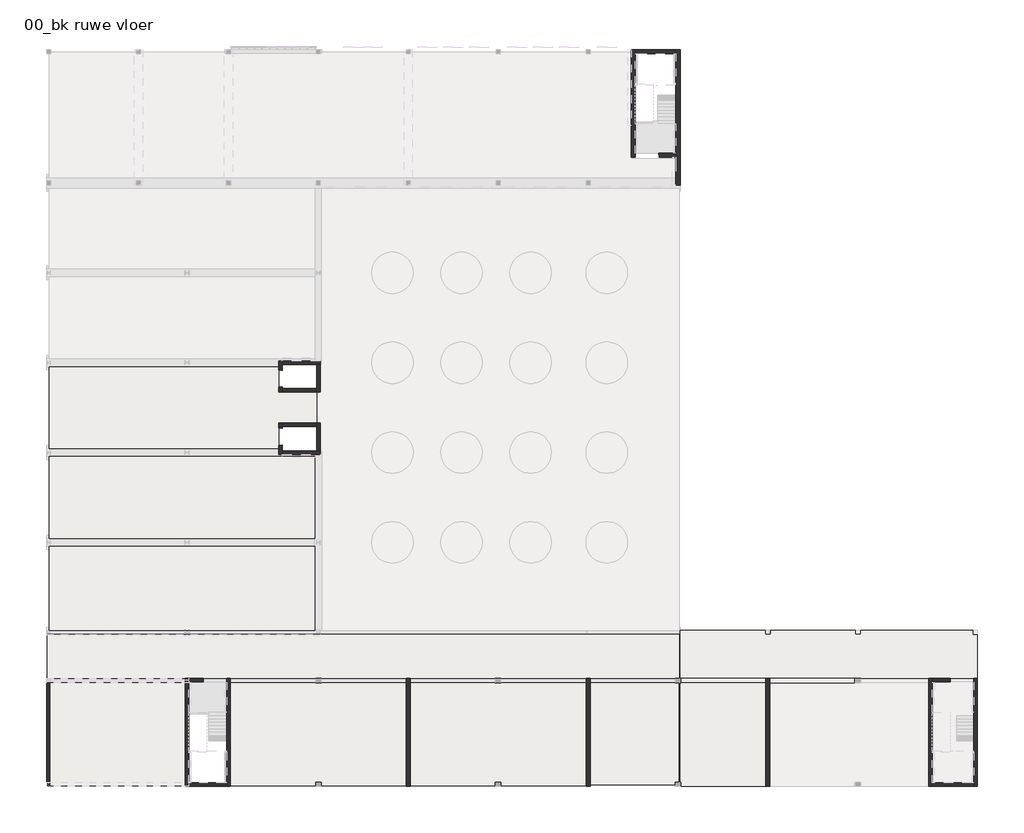
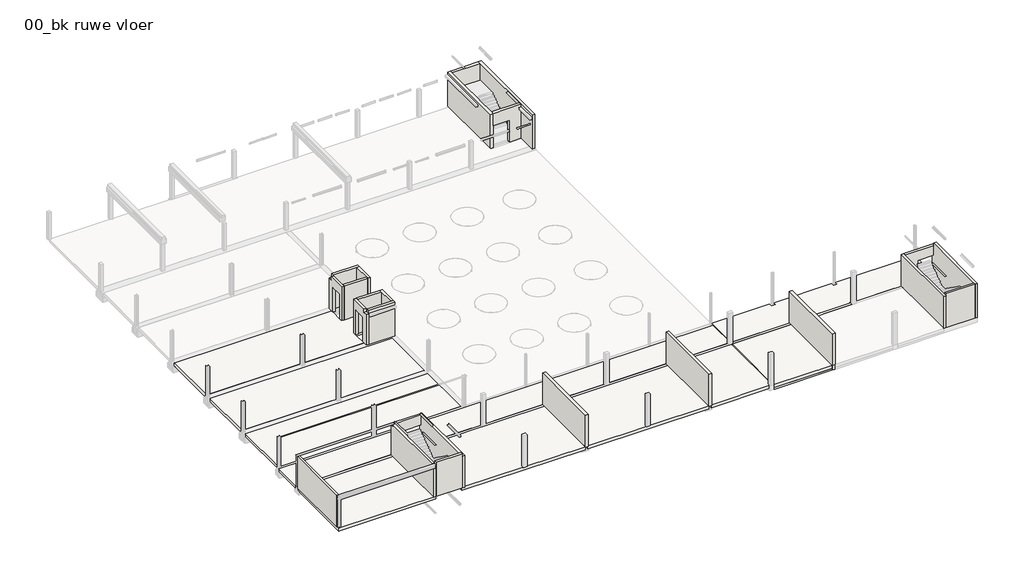
# One storey, part 1 of 6: 24 walls, 18 slabs.
"""IFC4 building model written with IfcOpenShell, lengths in millimetres."""

import ifcopenshell
import ifcopenshell.guid

model = None  # the IFC model being written
_history = None  # IfcOwnerHistory: only IFC2X3 demands one
_inside = {}  # id of a spatial element -> (the spatial element, [elements in it])
_under = {}  # id of a project, library or spatial element -> (it, [spatial elements below it])
_declared = {}  # id of a project -> (the project, [libraries it declares])
_typed = {}  # id of a type object -> (the type object, [elements of that type])
_made_of = {}  # id of a material, layer set ... -> (it, [elements and type objects made of it])


def new_model(schema):
    """Start an empty IFC model of exactly this schema.

    Asked for "IFC4X3", IfcOpenShell would pick the latest addendum, in which some entities
    have other attributes; the version numbers below select the first issue.
    IFC2X3 requires an IfcOwnerHistory on every rooted entity: one is made here for all.
    """
    global model, _history
    if schema == "IFC4X3":
        model = ifcopenshell.file(schema_version=(4, 3, 0, 0))
    else:
        model = ifcopenshell.file(schema=schema)
    _inside.clear()
    _under.clear()
    _declared.clear()
    _typed.clear()
    _made_of.clear()
    _history = None
    if model.schema == "IFC2X3":
        org = make("IfcOrganization", Name="unknown")
        user = make(
            "IfcPersonAndOrganization",
            ThePerson=make("IfcPerson", FamilyName="unknown"),
            TheOrganization=org,
        )
        app = make(
            "IfcApplication",
            ApplicationDeveloper=org,
            Version="unknown",
            ApplicationFullName="unknown",
            ApplicationIdentifier="unknown",
        )
        _history = make(
            "IfcOwnerHistory",
            OwningUser=user,
            OwningApplication=app,
            ChangeAction="ADDED",
            CreationDate=0,
        )
    return model


def make(cls, **values):
    """One entity of the class cls with the attributes given. An attribute that is None is left unset."""
    return model.create_entity(
        cls, **{name: value for name, value in values.items() if value is not None}
    )


def rooted(cls, **values):
    """An entity with a GlobalId (a new one), such as an element, a storey or a relation."""
    return make(cls, GlobalId=ifcopenshell.guid.new(), OwnerHistory=_history, **values)


def si_unit(unit_type, name, prefix=None):
    """IfcSIUnit, for example si_unit("LENGTHUNIT", "METRE", prefix="MILLI")."""
    return make("IfcSIUnit", UnitType=unit_type, Prefix=prefix, Name=name)


def assignment(units):
    """IfcUnitAssignment: the units of a project."""
    return None if units is None else make("IfcUnitAssignment", Units=units)


def point(xyz):
    """IfcCartesianPoint."""
    return None if xyz is None else make("IfcCartesianPoint", Coordinates=xyz)


def direction(xyz):
    """IfcDirection."""
    return None if xyz is None else make("IfcDirection", DirectionRatios=xyz)


def frame(location, z_axis=None, x_axis=None):
    """IfcAxis2Placement3D, a coordinate frame: its origin and axes. An axis left out is left unset."""
    return make(
        "IfcAxis2Placement3D",
        Location=point(location),
        Axis=direction(z_axis),
        RefDirection=direction(x_axis),
    )


def origin():
    """The frame at (0, 0, 0) with its axes left unset."""
    return frame((0.0, 0.0, 0.0))


def place(relative_to, where):
    """IfcLocalPlacement: puts the frame where relative to a parent placement (None: the world)."""
    return make(
        "IfcLocalPlacement", PlacementRelTo=relative_to, RelativePlacement=where
    )


def context(
    kind, dimensions, precision=None, world=None, true_north=None, identifier=None
):
    """IfcGeometricRepresentationContext, for example the 3D "Model" context."""
    return make(
        "IfcGeometricRepresentationContext",
        ContextIdentifier=identifier,
        ContextType=kind,
        CoordinateSpaceDimension=dimensions,
        Precision=precision,
        WorldCoordinateSystem=world,
        TrueNorth=true_north,
    )


def project(units=None, contexts=None):
    """IfcProject with its units and contexts."""
    return rooted(
        "IfcProject",
        Name="project",
        RepresentationContexts=contexts,
        UnitsInContext=assignment(units),
    )


def spatial(cls, under=None, at=None, **own):
    """A site, building, storey or space (cls), placed at a placement, below another one or the project."""
    s = rooted(cls, ObjectPlacement=at, **own)
    if under is not None:
        _under.setdefault(under.id(), (under, []))[1].append(s)
    return s


def polyline(points):
    """IfcPolyline through the points."""
    return make("IfcPolyline", Points=[point(p) for p in points])


def outline(outer, holes=None, kind="AREA"):
    """IfcArbitraryClosedProfileDef: a profile drawn as a closed curve; with holes, ...WithVoids."""
    if holes is None:
        return make("IfcArbitraryClosedProfileDef", ProfileType=kind, OuterCurve=outer)
    return make(
        "IfcArbitraryProfileDefWithVoids",
        ProfileType=kind,
        OuterCurve=outer,
        InnerCurves=holes,
    )


def extrude(swept, where, along, depth):
    """IfcExtrudedAreaSolid: the profile swept, set in the frame where, extruded along a direction by depth."""
    return make(
        "IfcExtrudedAreaSolid",
        SweptArea=swept,
        Position=where,
        ExtrudedDirection=direction(along),
        Depth=depth,
    )


def faces_of(points, faces, orient=None, outer=None):
    """IfcFace entities. A face is a list of loops; a loop is a list of indices into points, from 0.

    orient and outer hold one flag for each loop. By default every Orientation is true, the
    first loop of a face is its IfcFaceOuterBound and the others are IfcFaceBound.
    """
    made = []
    for i, loops in enumerate(faces):
        bounds = []
        for j, loop in enumerate(loops):
            is_outer = j == 0 if outer is None else outer[i][j]
            bounds.append(
                make(
                    "IfcFaceOuterBound" if is_outer else "IfcFaceBound",
                    Bound=make("IfcPolyLoop", Polygon=[points[k] for k in loop]),
                    Orientation=True if orient is None else orient[i][j],
                )
            )
        made.append(make("IfcFace", Bounds=bounds))
    return made


def faceted_brep(points, faces, orient=None, outer=None, voids=None):
    """IfcFacetedBrep: a solid bounded by flat faces; with voids (closed shells), ...WithVoids."""
    shared = [point(p) for p in points]
    hull = make("IfcClosedShell", CfsFaces=faces_of(shared, faces, orient, outer))
    if voids is None:
        return make("IfcFacetedBrep", Outer=hull)
    return make(
        "IfcFacetedBrepWithVoids",
        Outer=hull,
        Voids=[
            make(cls, CfsFaces=faces_of(shared, fs, o, b)) for cls, fs, o, b in voids
        ],
    )


def shape(context_of_items, identifier, shape_type, items):
    """IfcShapeRepresentation: the items that make up one representation, for example the "Body"."""
    return make(
        "IfcShapeRepresentation",
        ContextOfItems=context_of_items,
        RepresentationIdentifier=identifier,
        RepresentationType=shape_type,
        Items=items,
    )


def made_of(thing, what):
    """Note that an element or type object is made of a material, layer set ...; save() writes the relation."""
    if what is not None:
        _made_of.setdefault(what.id(), (what, []))[1].append(thing)
    return thing


def element(
    cls,
    number,
    at=None,
    inside=None,
    cuts=None,
    type_object=None,
    material=None,
    context=None,
    identifier="Body",
    shape_type=None,
    held_by="IfcProductDefinitionShape",
    body=None,
    shapes=None,
    **own,
):
    """One element of the class cls, such as IfcWall. Its Tag is "e" and its number.

    at: its placement. inside: the storey or other place that contains it. cuts: it is an
    opening in that element (IfcRelVoidsElement). A single representation is given by context,
    identifier, shape_type and body (its items); several are given by shapes. held_by: the class
    of the entity that holds the representations. save() writes the other relations.
    """
    e = rooted(cls, Tag="e%d" % number, ObjectPlacement=at, **own)
    if body is not None:
        shapes = [shape(context, identifier, shape_type, body)]
    if shapes is not None:
        e.Representation = make(held_by, Representations=shapes)
    if inside is not None:
        _inside.setdefault(inside.id(), (inside, []))[1].append(e)
    if cuts is not None:
        rooted(
            "IfcRelVoidsElement", RelatingBuildingElement=cuts, RelatedOpeningElement=e
        )
    if type_object is not None:
        _typed.setdefault(type_object.id(), (type_object, []))[1].append(e)
    return made_of(e, material)


def aggregate(whole, parts):
    """IfcRelAggregates: a whole, such as a stair, and the parts it consists of."""
    return rooted("IfcRelAggregates", RelatingObject=whole, RelatedObjects=parts)


def save(model, path):
    """Write the relations noted so far, then the file.

    IfcRelAggregates (storeys below a building ...), IfcRelContainedInSpatialStructure (elements
    in a storey), IfcRelDefinesByType, IfcRelAssociatesMaterial and IfcRelDeclares: one each for
    every whole, place, type object, material and project.
    """
    for whole, parts in _under.values():
        aggregate(whole, parts)
    for where, things in _inside.values():
        rooted(
            "IfcRelContainedInSpatialStructure",
            RelatedElements=things,
            RelatingStructure=where,
        )
    for kind, things in _typed.values():
        rooted("IfcRelDefinesByType", RelatedObjects=things, RelatingType=kind)
    for what, things in _made_of.values():
        rooted("IfcRelAssociatesMaterial", RelatedObjects=things, RelatingMaterial=what)
    for by, libraries in _declared.values():
        rooted("IfcRelDeclares", RelatingContext=by, RelatedDefinitions=libraries)
    model.write(path)


model = new_model("IFC4")

# Units and contexts
model_context = context("Model", 3, world=origin())
ifc_project = project(units=[si_unit("LENGTHUNIT", "METRE", prefix="MILLI")], contexts=[model_context])

# Site, building, storey
site = spatial("IfcSite", under=ifc_project)
building = spatial("IfcBuilding", under=site)
storey = spatial("IfcBuildingStorey", under=building, Name="00_bk ruwe vloer", Elevation=-70.0)

# Slabs
placement = place(None, origin())
element("IfcSlab", 1, ObjectType="NLRS_23_FL_isolatieplaatvloer 320_gen_rsf", at=placement, inside=storey, context=model_context, shape_type="Brep", body=[
    faceted_brep([(52150.0, 7650.0, -390.0), (52150.0, 11150.0, -390.0), (58300.0, 11150.0, -390.0), (58300.0, 10850.0, -390.0), (58700.0, 10850.0, -390.0), (58700.0, 11150.0, -390.0), (64800.0, 11150.0, -390.0), (64800.0, 10850.0, -390.0), (65200.0, 10850.0, -390.0), (65200.0, 11150.0, -390.0), (73300.0, 11150.0, -390.0), (73300.0, 10800.0, -390.0), (73650.0, 10800.0, -390.0), (73650.0, 7650.0, -390.0), (65250.0, 7650.0, -390.0), (65250.0, 7700.0, -390.0), (64750.0, 7700.0, -390.0), (64750.0, 7650.0, -390.0), (52150.0, 7650.0, -70.0), (64750.0, 7650.0, -70.0), (64750.0, 7700.0, -70.0), (65250.0, 7700.0, -70.0), (65250.0, 7650.0, -70.0), (73650.0, 7650.0, -70.0), (73650.0, 10800.0, -70.0), (73300.0, 10800.0, -70.0), (73300.0, 11150.0, -70.0), (65200.0, 11150.0, -70.0), (65200.0, 10850.0, -70.0), (64800.0, 10850.0, -70.0), (64800.0, 11150.0, -70.0), (58700.0, 11150.0, -70.0), (58700.0, 10850.0, -70.0), (58300.0, 10850.0, -70.0), (58300.0, 11150.0, -70.0), (52150.0, 11150.0, -70.0), (52150.0, 10850.0, -70.0)], [[[0, 1, 2, 3, 4, 5, 6, 7, 8, 9, 10, 11, 12, 13, 14, 15, 16, 17]], [[18, 19, 20, 21, 22, 23, 24, 25, 26, 27, 28, 29, 30, 31, 32, 33, 34, 35, 36]], [[1, 0, 18, 36, 35]], [[10, 9, 27, 26]], [[13, 12, 24, 23]], [[0, 17, 19, 18]], [[14, 13, 23, 22]], [[15, 14, 22, 21]], [[16, 15, 21, 20]], [[17, 16, 20, 19]], [[2, 1, 35, 34]], [[3, 2, 34, 33]], [[4, 3, 33, 32]], [[5, 4, 32, 31]], [[6, 5, 31, 30]], [[7, 6, 30, 29]], [[8, 7, 29, 28]], [[9, 8, 28, 27]], [[11, 10, 26, 25]], [[12, 11, 25, 24]]]),
])
element("IfcSlab", 2, ObjectType="NLRS_23_FL_breedplaat 320_gen_rsf", at=placement, inside=storey, context=model_context, shape_type="Brep", body=[
    faceted_brep([(6410.0, 7350.0, -390.0), (16375.0, 7350.0, -390.0), (16625.0, 7350.0, -390.0), (16625.0, 150.0, -390.0), (16625.0, -90.0, -390.0), (6650.0, -90.0, -390.0), (6410.0, -90.0, -390.0), (6410.0, 7150.0, -390.0), (16400.0, 125.0, -390.0), (16400.0, 7175.0, -390.0), (6625.0, 7175.0, -390.0), (6625.0, 125.0, -390.0), (16625.0, 7350.0, -70.0), (6410.0, 7350.0, -70.0), (6410.0, -90.0, -70.0), (6650.0, -90.0, -70.0), (16625.0, -90.0, -70.0), (16625.0, 150.0, -70.0), (6625.0, 7175.0, -330.0), (16400.0, 7175.0, -330.0), (16400.0, 125.0, -330.0), (6625.0, 125.0, -330.0)], [[[0, 1, 2, 3, 4, 5, 6, 7], [8, 9, 10, 11]], [[12, 13, 14, 15, 16, 17]], [[2, 1, 0, 13, 12]], [[4, 3, 2, 12, 17, 16]], [[6, 5, 4, 16, 15, 14]], [[0, 7, 6, 14, 13]], [[18, 19, 20, 21]], [[20, 19, 9, 8]], [[21, 20, 8, 11]], [[18, 21, 11, 10]], [[19, 18, 10, 9]]]),
])
element("IfcSlab", 3, ObjectType="NLRS_23_FL_breedplaat 320_gen_rsf", at=placement, inside=storey, context=model_context, shape_type="Brep", body=[
    faceted_brep([(52090.0, 10850.0, -390.0), (52090.0, 10650.0, -390.0), (52090.0, 7850.0, -390.0), (52090.0, 7650.0, -390.0), (19375.0, 7650.0, -390.0), (16625.0, 7650.0, -390.0), (16375.0, 7650.0, -390.0), (6410.0, 7650.0, -390.0), (6410.0, 7850.0, -390.0), (6410.0, 10650.0, -390.0), (6410.0, 10850.0, -390.0), (51875.0, 7825.0, -390.0), (51875.0, 10675.0, -390.0), (6625.0, 10675.0, -390.0), (6625.0, 7825.0, -390.0), (52090.0, 7650.0, -70.0), (52090.0, 10850.0, -70.0), (6410.0, 10850.0, -70.0), (6410.0, 7650.0, -70.0), (16625.0, 7650.0, -70.0), (19375.0, 7650.0, -70.0), (6625.0, 10675.0, -330.0), (51875.0, 10675.0, -330.0), (51875.0, 7825.0, -330.0), (6625.0, 7825.0, -330.0)], [[[0, 1, 2, 3, 4, 5, 6, 7, 8, 9, 10], [11, 12, 13, 14]], [[15, 16, 17, 18, 19, 20]], [[3, 2, 1, 0, 16, 15]], [[7, 6, 5, 4, 3, 15, 20, 19, 18]], [[10, 9, 8, 7, 18, 17]], [[0, 10, 17, 16]], [[21, 22, 23, 24]], [[23, 22, 12, 11]], [[24, 23, 11, 14]], [[21, 24, 14, 13]], [[22, 21, 13, 12]]]),
])
element("IfcSlab", 4, ObjectType="NLRS_23_FL_isolatieplaatvloer 320_gen_rsf", at=placement, inside=storey, context=model_context, shape_type="Brep", body=[
    faceted_brep([(25750.0, 17200.0, -390.0), (25750.0, 11350.0, -390.0), (25750.0, 11150.0, -390.0), (6550.0, 11150.0, -390.0), (6550.0, 11350.0, -390.0), (6550.0, 17000.0, -390.0), (6550.0, 17200.0, -390.0), (25500.0, 17200.0, -390.0), (25550.0, 17200.0, -390.0), (25700.0, 17200.0, -390.0), (25750.0, 17200.0, -70.0), (25700.0, 17200.0, -70.0), (6550.0, 17200.0, -70.0), (6550.0, 11150.0, -70.0), (25750.0, 11150.0, -70.0)], [[[0, 1, 2, 3, 4, 5, 6, 7, 8, 9]], [[10, 11, 12, 13, 14]], [[2, 1, 0, 10, 14]], [[3, 2, 14, 13]], [[6, 5, 4, 3, 13, 12]], [[0, 9, 8, 7, 6, 12, 11, 10]]]),
])
element("IfcSlab", 5, ObjectType="NLRS_23_FL_isolatieplaatvloer 320_gen_rsf", at=placement, inside=storey, context=model_context, shape_type="Brep", body=[
    faceted_brep([(25750.0, 23700.0, -390.0), (25750.0, 17800.0, -390.0), (25700.0, 17800.0, -390.0), (25550.0, 17800.0, -390.0), (25500.0, 17800.0, -390.0), (6550.0, 17800.0, -390.0), (6550.0, 18000.0, -390.0), (6550.0, 23500.0, -390.0), (6550.0, 23700.0, -390.0), (25500.0, 23700.0, -390.0), (25550.0, 23700.0, -390.0), (25700.0, 23700.0, -390.0), (25750.0, 23700.0, -70.0), (25700.0, 23700.0, -70.0), (6550.0, 23700.0, -70.0), (6550.0, 17800.0, -70.0), (25700.0, 17800.0, -70.0), (25750.0, 17800.0, -70.0)], [[[0, 1, 2, 3, 4, 5, 6, 7, 8, 9, 10, 11]], [[12, 13, 14, 15, 16, 17]], [[1, 0, 12, 17]], [[5, 4, 3, 2, 1, 17, 16, 15]], [[8, 7, 6, 5, 15, 14]], [[0, 11, 10, 9, 8, 14, 13, 12]]]),
])
element("IfcSlab", 6, ObjectType="NLRS_23_FL_isolatieplaatvloer 320_gen_rsf", at=placement, inside=storey, context=model_context, shape_type="Brep", body=[
    faceted_brep([(23125.0, 30200.0, -390.0), (23125.0, 30000.0, -390.0), (23125.0, 28475.0, -390.0), (23375.0, 28475.0, -390.0), (25875.0, 28475.0, -390.0), (25875.0, 28375.0, -390.0), (25875.0, 26125.0, -390.0), (25875.0, 26025.0, -390.0), (23375.0, 26025.0, -390.0), (23125.0, 26025.0, -390.0), (23125.0, 24500.0, -390.0), (23125.0, 24300.0, -390.0), (6550.0, 24300.0, -390.0), (6550.0, 24500.0, -390.0), (6550.0, 30000.0, -390.0), (6550.0, 30200.0, -390.0), (23125.0, 30200.0, -70.0), (6550.0, 30200.0, -70.0), (6550.0, 24300.0, -70.0), (23125.0, 24300.0, -70.0), (23125.0, 26025.0, -70.0), (23375.0, 26025.0, -70.0), (25875.0, 26025.0, -70.0), (25875.0, 28475.0, -70.0), (23375.0, 28475.0, -70.0), (23125.0, 28475.0, -70.0)], [[[0, 1, 2, 3, 4, 5, 6, 7, 8, 9, 10, 11, 12, 13, 14, 15]], [[16, 17, 18, 19, 20, 21, 22, 23, 24, 25]], [[2, 1, 0, 16, 25]], [[12, 11, 19, 18]], [[15, 14, 13, 12, 18, 17]], [[0, 15, 17, 16]], [[4, 3, 2, 25, 24, 23]], [[7, 6, 5, 4, 23, 22]], [[9, 8, 7, 22, 21, 20]], [[11, 10, 9, 20, 19]]]),
])
element("IfcSlab", 7, ObjectType="NLRS_23_FL_breedplaat 320_gen_rsf", at=placement, inside=storey, context=model_context, shape_type="Brep", body=[
    faceted_brep([(32350.0, 7350.0, -390.0), (32350.0, 150.0, -390.0), (32350.0, -90.0, -390.0), (19375.0, -90.0, -390.0), (19375.0, 150.0, -390.0), (19375.0, 7350.0, -390.0), (32175.0, 125.0, -390.0), (32175.0, 7175.0, -390.0), (19600.0, 7175.0, -390.0), (19600.0, 125.0, -390.0), (32350.0, -90.0, -70.0), (32350.0, 150.0, -70.0), (32350.0, 7350.0, -70.0), (19375.0, 7350.0, -70.0), (19375.0, 150.0, -70.0), (19375.0, -90.0, -70.0), (19600.0, 7175.0, -330.0), (32175.0, 7175.0, -330.0), (32175.0, 125.0, -330.0), (19600.0, 125.0, -330.0)], [[[0, 1, 2, 3, 4, 5], [6, 7, 8, 9]], [[10, 11, 12, 13, 14, 15]], [[2, 1, 0, 12, 11, 10]], [[3, 2, 10, 15]], [[5, 4, 3, 15, 14, 13]], [[0, 5, 13, 12]], [[16, 17, 18, 19]], [[18, 17, 7, 6]], [[19, 18, 6, 9]], [[16, 19, 9, 8]], [[17, 16, 8, 7]]]),
])
element("IfcSlab", 8, ObjectType="NLRS_23_FL_breedplaat 320_gen_rsf", at=placement, inside=storey, context=model_context, shape_type="Brep", body=[
    faceted_brep([(45350.0, 7350.0, -390.0), (45350.0, 7150.0, -390.0), (45350.0, 150.0, -390.0), (45350.0, -90.0, -390.0), (32650.0, -90.0, -390.0), (32650.0, 150.0, -390.0), (32650.0, 7150.0, -390.0), (32650.0, 7350.0, -390.0), (45175.0, 125.0, -390.0), (45175.0, 7175.0, -390.0), (32825.0, 7175.0, -390.0), (32825.0, 125.0, -390.0), (45350.0, -90.0, -70.0), (45350.0, 150.0, -70.0), (45350.0, 7350.0, -70.0), (32650.0, 7350.0, -70.0), (32650.0, 150.0, -70.0), (32650.0, -90.0, -70.0), (32825.0, 7175.0, -330.0), (45175.0, 7175.0, -330.0), (45175.0, 125.0, -330.0), (32825.0, 125.0, -330.0)], [[[0, 1, 2, 3, 4, 5, 6, 7], [8, 9, 10, 11]], [[12, 13, 14, 15, 16, 17]], [[3, 2, 1, 0, 14, 13, 12]], [[4, 3, 12, 17]], [[7, 6, 5, 4, 17, 16, 15]], [[0, 7, 15, 14]], [[18, 19, 20, 21]], [[20, 19, 9, 8]], [[21, 20, 8, 11]], [[18, 21, 11, 10]], [[19, 18, 10, 9]]]),
])
element("IfcSlab", 9, ObjectType="NLRS_23_FL_breedplaat 320_gen_rsf", at=placement, inside=storey, context=model_context, shape_type="Brep", body=[
    faceted_brep([(52050.0, 7350.0, -390.0), (52050.0, 7150.0, -390.0), (52050.0, 150.0, -390.0), (52050.0, -50.0, -390.0), (51750.0, -50.0, -390.0), (45650.0, -50.0, -390.0), (45650.0, 150.0, -390.0), (45650.0, 7150.0, -390.0), (45650.0, 7350.0, -390.0), (51875.0, 125.0, -390.0), (51875.0, 7175.0, -390.0), (45825.0, 7175.0, -390.0), (45825.0, 125.0, -390.0), (52050.0, -50.0, -70.0), (52050.0, 150.0, -70.0), (52050.0, 7350.0, -70.0), (45650.0, 7350.0, -70.0), (45650.0, 150.0, -70.0), (45650.0, -50.0, -70.0), (51750.0, -50.0, -70.0), (45825.0, 7175.0, -330.0), (51875.0, 7175.0, -330.0), (51875.0, 125.0, -330.0), (45825.0, 125.0, -330.0)], [[[0, 1, 2, 3, 4, 5, 6, 7, 8], [9, 10, 11, 12]], [[13, 14, 15, 16, 17, 18, 19]], [[3, 2, 1, 0, 15, 14, 13]], [[5, 4, 3, 13, 19, 18]], [[8, 7, 6, 5, 18, 17, 16]], [[0, 8, 16, 15]], [[20, 21, 22, 23]], [[22, 21, 10, 9]], [[23, 22, 9, 12]], [[20, 23, 12, 11]], [[21, 20, 11, 10]]]),
])
element("IfcSlab", 10, ObjectType="NLRS_23_FL_isolatieplaatvloer 320_gen_rsf", at=placement, inside=storey, context=model_context, shape_type="SweptSolid", body=[
    extrude(outline(polyline([(58350.0, 7350.0), (58350.0, -150.0), (52250.0, -150.0), (52250.0, 150.0), (52150.0, 150.0), (52150.0, 7350.0), (58350.0, 7350.0)])), frame((0.0, 0.0, -390.0), z_axis=(0.0, 0.0, 1.0), x_axis=(1.0, 0.0, 0.0)), (0.0, 0.0, 1.0), 320.0),
])
element("IfcSlab", 11, ObjectType="NLRS_23_FL_beton ihwg vloeraanstort 520_gen_rsf", at=placement, inside=storey, context=model_context, shape_type="Brep", body=[
    faceted_brep([(64750.0, 7650.0, -590.0), (64750.0, 7350.0, -590.0), (58650.0, 7350.0, -590.0), (58650.0, -150.0, -590.0), (58350.0, -150.0, -590.0), (58350.0, 7350.0, -590.0), (52150.0, 7350.0, -590.0), (52150.0, 7650.0, -590.0), (64750.0, 7650.0, -70.0), (52200.0, 7650.0, -70.0), (52150.0, 7650.0, -70.0), (52150.0, 7350.0, -70.0), (52200.0, 7350.0, -70.0), (58350.0, 7350.0, -70.0), (58350.0, -150.0, -70.0), (58650.0, -150.0, -70.0), (58650.0, 7350.0, -70.0), (64750.0, 7350.0, -70.0), (52150.0, 7350.0, -390.0), (52150.0, 7650.0, -390.0)], [[[0, 1, 2, 3, 4, 5, 6, 7]], [[8, 9, 10, 11, 12, 13, 14, 15, 16, 17]], [[1, 0, 8, 17]], [[2, 1, 17, 16]], [[3, 2, 16, 15]], [[4, 3, 15, 14]], [[5, 4, 14, 13]], [[6, 5, 13, 12, 11, 18]], [[7, 6, 18, 11, 10, 19]], [[0, 7, 19, 10, 9, 8]]]),
])
element("IfcSlab", 12, ObjectType="NLRS_23_FL_isolatie isolatieplaatvloer 200_gen_rsf", at=placement, inside=storey, context=model_context, shape_type="Brep", body=[
    faceted_brep([(52150.0, 7650.0, -590.0), (52150.0, 7800.0, -590.0), (52150.0, 10750.0, -590.0), (52150.0, 11150.0, -590.0), (58300.0, 11150.0, -590.0), (58300.0, 10850.0, -590.0), (58700.0, 10850.0, -590.0), (58700.0, 11150.0, -590.0), (64800.0, 11150.0, -590.0), (64800.0, 10850.0, -590.0), (65200.0, 10850.0, -590.0), (65200.0, 11150.0, -590.0), (73300.0, 11150.0, -590.0), (73300.0, 10800.0, -590.0), (73650.0, 10800.0, -590.0), (73650.0, 7650.0, -590.0), (65250.0, 7650.0, -590.0), (65250.0, 7700.0, -590.0), (64750.0, 7700.0, -590.0), (64750.0, 7650.0, -590.0), (52150.0, 7650.0, -390.0), (64750.0, 7650.0, -390.0), (64750.0, 7700.0, -390.0), (65250.0, 7700.0, -390.0), (65250.0, 7650.0, -390.0), (73650.0, 7650.0, -390.0), (73650.0, 10800.0, -390.0), (73300.0, 10800.0, -390.0), (73300.0, 11150.0, -390.0), (65200.0, 11150.0, -390.0), (65200.0, 10850.0, -390.0), (64800.0, 10850.0, -390.0), (64800.0, 11150.0, -390.0), (58700.0, 11150.0, -390.0), (58700.0, 10850.0, -390.0), (58300.0, 10850.0, -390.0), (58300.0, 11150.0, -390.0), (52150.0, 11150.0, -390.0), (52150.0, 10850.0, -390.0), (52150.0, 10650.0, -390.0), (52150.0, 7850.0, -390.0)], [[[0, 1, 2, 3, 4, 5, 6, 7, 8, 9, 10, 11, 12, 13, 14, 15, 16, 17, 18, 19]], [[20, 21, 22, 23, 24, 25, 26, 27, 28, 29, 30, 31, 32, 33, 34, 35, 36, 37, 38, 39, 40]], [[3, 2, 1, 0, 20, 40, 39, 38, 37]], [[12, 11, 29, 28]], [[15, 14, 26, 25]], [[0, 19, 21, 20]], [[16, 15, 25, 24]], [[17, 16, 24, 23]], [[18, 17, 23, 22]], [[19, 18, 22, 21]], [[4, 3, 37, 36]], [[5, 4, 36, 35]], [[6, 5, 35, 34]], [[7, 6, 34, 33]], [[8, 7, 33, 32]], [[9, 8, 32, 31]], [[10, 9, 31, 30]], [[11, 10, 30, 29]], [[13, 12, 28, 27]], [[14, 13, 27, 26]]]),
])
element("IfcSlab", 13, ObjectType="NLRS_23_FL_isolatie isolatieplaatvloer 200_gen_rsf", at=placement, inside=storey, context=model_context, shape_type="Brep", body=[
    faceted_brep([(58350.0, 7350.0, -590.0), (58350.0, -150.0, -590.0), (52250.0, -150.0, -590.0), (52250.0, 150.0, -590.0), (52150.0, 150.0, -590.0), (52150.0, 250.0, -590.0), (52150.0, 7200.0, -590.0), (52150.0, 7350.0, -590.0), (58350.0, 7350.0, -390.0), (52150.0, 7350.0, -390.0), (52150.0, 7150.0, -390.0), (52150.0, 150.0, -390.0), (52250.0, 150.0, -390.0), (52250.0, -150.0, -390.0), (58350.0, -150.0, -390.0)], [[[0, 1, 2, 3, 4, 5, 6, 7]], [[8, 9, 10, 11, 12, 13, 14]], [[1, 0, 8, 14]], [[2, 1, 14, 13]], [[7, 6, 5, 4, 11, 10, 9]], [[0, 7, 9, 8]], [[3, 2, 13, 12]], [[4, 3, 12, 11]]]),
])
element("IfcSlab", 14, ObjectType="NLRS_23_FL_breedplaat schil 60_gen_rsf", at=placement, inside=storey, context=model_context, shape_type="SweptSolid", body=[
    extrude(outline(polyline([(16400.0, 7175.0), (16400.0, 125.0), (6625.0, 125.0), (6625.0, 7175.0), (16400.0, 7175.0)])), frame((0.0, 0.0, -390.0), z_axis=(0.0, 0.0, 1.0), x_axis=(1.0, 0.0, 0.0)), (0.0, 0.0, 1.0), 60.0),
])
element("IfcSlab", 15, ObjectType="NLRS_23_FL_breedplaat schil 60_gen_rsf", at=placement, inside=storey, context=model_context, shape_type="SweptSolid", body=[
    extrude(outline(polyline([(32175.0, 7175.0), (32175.0, 125.0), (19600.0, 125.0), (19600.0, 7175.0), (32175.0, 7175.0)])), frame((0.0, 0.0, -390.0), z_axis=(0.0, 0.0, 1.0), x_axis=(1.0, 0.0, 0.0)), (0.0, 0.0, 1.0), 60.0),
])
element("IfcSlab", 16, ObjectType="NLRS_23_FL_breedplaat schil 60_gen_rsf", at=placement, inside=storey, context=model_context, shape_type="SweptSolid", body=[
    extrude(outline(polyline([(45175.0, 7175.0), (45175.0, 125.0), (32825.0, 125.0), (32825.0, 7175.0), (45175.0, 7175.0)])), frame((0.0, 0.0, -390.0), z_axis=(0.0, 0.0, 1.0), x_axis=(1.0, 0.0, 0.0)), (0.0, 0.0, 1.0), 60.0),
])
element("IfcSlab", 17, ObjectType="NLRS_23_FL_breedplaat schil 60_gen_rsf", at=placement, inside=storey, context=model_context, shape_type="SweptSolid", body=[
    extrude(outline(polyline([(51875.0, 7175.0), (51875.0, 125.0), (45825.0, 125.0), (45825.0, 7175.0), (51875.0, 7175.0)])), frame((0.0, 0.0, -390.0), z_axis=(0.0, 0.0, 1.0), x_axis=(1.0, 0.0, 0.0)), (0.0, 0.0, 1.0), 60.0),
])
element("IfcSlab", 18, ObjectType="NLRS_23_FL_breedplaat schil 60_gen_rsf", at=placement, inside=storey, context=model_context, shape_type="SweptSolid", body=[
    extrude(outline(polyline([(51875.0, 10675.0), (51875.0, 7825.0), (6625.0, 7825.0), (6625.0, 10675.0), (51875.0, 10675.0)])), frame((0.0, 0.0, -390.0), z_axis=(0.0, 0.0, 1.0), x_axis=(1.0, 0.0, 0.0)), (0.0, 0.0, 1.0), 60.0),
])

# Walls
element("IfcWall", 19, ObjectType="NLRS_22_WA_beton ihw 250_gen_rsf", at=placement, inside=storey, context=model_context, shape_type="Brep", body=[
    faceted_brep([(19625.0, -150.0, -70.0), (19625.0, 7650.0, -70.0), (19625.0, 7650.0, 3470.0), (19625.0, -150.0, 3470.0), (19375.0, -150.0, -70.0), (19375.0, -150.0, 3470.0), (19375.0, 7400.0, 3470.0), (19375.0, 7650.0, 3470.0), (19375.0, 7650.0, 2370.0), (19375.0, 7650.0, -70.0), (19375.0, 7350.0, -70.0), (19375.0, 100.0, -70.0), (19375.0, -90.0, -70.0)], [[[0, 1, 2, 3]], [[4, 5, 6, 7, 8, 9, 10, 11, 12]], [[1, 0, 4, 12, 11, 10, 9]], [[2, 1, 9, 8, 7]], [[3, 2, 7, 6, 5]], [[0, 3, 5, 4]]]),
])
element("IfcWall", 20, ObjectType="NLRS_22_WA_beton ihw 250_gen_rsf", at=placement, inside=storey, context=model_context, shape_type="Brep", body=[
    faceted_brep([(16625.0, -150.0, -70.0), (16625.0, -90.0, -70.0), (16625.0, 100.0, -70.0), (16625.0, 7350.0, -70.0), (16625.0, 7400.0, -70.0), (16625.0, 7650.0, -70.0), (16625.0, 7650.0, 3320.0), (16625.0, 7330.0, 3320.0), (16625.0, 7330.0, 3470.0), (16625.0, 170.0, 3470.0), (16625.0, 170.0, 3090.0), (16625.0, -150.0, 3090.0), (16375.0, -150.0, -70.0), (16375.0, -150.0, 3090.0), (16375.0, 170.0, 3090.0), (16375.0, 170.0, 3470.0), (16375.0, 7330.0, 3470.0), (16375.0, 7330.0, 3320.0), (16375.0, 7650.0, 3320.0), (16375.0, 7650.0, -70.0)], [[[0, 1, 2, 3, 4, 5, 6, 7, 8, 9, 10, 11]], [[12, 13, 14, 15, 16, 17, 18, 19]], [[5, 4, 3, 2, 1, 0, 12, 19]], [[6, 5, 19, 18]], [[9, 8, 16, 15]], [[0, 11, 13, 12]], [[10, 9, 15, 14]], [[11, 10, 14, 13]], [[7, 6, 18, 17]], [[8, 7, 17, 16]]]),
])
element("IfcWall", 21, ObjectType="NLRS_22_WA_kalkzandsteen CS20 300_gen_rsf", at=placement, inside=storey, context=model_context, shape_type="SweptSolid", body=[
    extrude(outline(polyline([(32650.0, 7650.0), (32650.0, -150.0), (32350.0, -150.0), (32350.0, 7650.0), (32650.0, 7650.0)])), frame((0.0, 0.0, -70.0), z_axis=(0.0, 0.0, 1.0), x_axis=(1.0, 0.0, 0.0)), (0.0, 0.0, 1.0), 3540.0),
])
element("IfcWall", 22, ObjectType="NLRS_22_WA_kalkzandsteen CS20 300_gen_rsf", at=placement, inside=storey, context=model_context, shape_type="SweptSolid", body=[
    extrude(outline(polyline([(45650.0, 7650.0), (45650.0, -150.0), (45350.0, -150.0), (45350.0, 7650.0), (45650.0, 7650.0)])), frame((0.0, 0.0, -70.0), z_axis=(0.0, 0.0, 1.0), x_axis=(1.0, 0.0, 0.0)), (0.0, 0.0, 1.0), 3540.0),
])
element("IfcWall", 23, ObjectType="NLRS_22_WA_kalkzandsteen CS20 300_gen_rsf", at=placement, inside=storey, context=model_context, shape_type="SweptSolid", body=[
    extrude(outline(polyline([(58650.0, 7650.0), (58650.0, -150.0), (58350.0, -150.0), (58350.0, 7650.0), (58650.0, 7650.0)])), frame((0.0, 0.0, -70.0), z_axis=(0.0, 0.0, 1.0), x_axis=(1.0, 0.0, 0.0)), (0.0, 0.0, 1.0), 3540.0),
])
element("IfcWall", 24, ObjectType="NLRS_21_WA_beton ihw 250_gen_rsf", at=placement, inside=storey, context=model_context, shape_type="Brep", body=[
    faceted_brep([(73650.0, -150.0, -70.0), (73650.0, 7650.0, -70.0), (73650.0, 7650.0, 3470.0), (73650.0, 7400.0, 3470.0), (73650.0, 7400.0, 3730.0), (73650.0, -150.0, 3730.0), (73400.0, -150.0, -70.0), (73400.0, -150.0, 3730.0), (73400.0, 100.0, 3730.0), (73400.0, 7400.0, 3730.0), (73400.0, 7400.0, 3470.0), (73400.0, 7650.0, 3470.0), (73400.0, 7650.0, 2370.0), (73400.0, 7650.0, -70.0), (73400.0, 7400.0, -70.0), (73400.0, 100.0, -70.0)], [[[0, 1, 2, 3, 4, 5]], [[6, 7, 8, 9, 10, 11, 12, 13, 14, 15]], [[1, 0, 6, 15, 14, 13]], [[2, 1, 13, 12, 11]], [[5, 4, 9, 8, 7]], [[0, 5, 7, 6]], [[3, 2, 11, 10]], [[4, 3, 10, 9]]]),
])
element("IfcWall", 25, ObjectType="NLRS_21_WA_kalkzandsteen CS12 214_gen_rsf", at=placement, inside=storey, context=model_context, shape_type="SweptSolid", body=[
    extrude(outline(polyline([(6564.0, 7330.0), (6564.0, 170.0), (6350.0, 170.0), (6350.0, 7330.0), (6564.0, 7330.0)])), frame((0.0, 0.0, -70.0), z_axis=(0.0, 0.0, 1.0), x_axis=(1.0, 0.0, 0.0)), (0.0, 0.0, 1.0), 3540.0),
])
element("IfcWall", 26, ObjectType="NLRS_21_WA_beton ihw 250_gen_rsf", at=placement, inside=storey, context=model_context, shape_type="Brep", body=[
    faceted_brep([(16625.0, -150.0, -70.0), (19375.0, -150.0, -70.0), (19375.0, -150.0, 3470.0), (19375.0, -150.0, 3730.0), (16625.0, -150.0, 3730.0), (16625.0, -150.0, 3470.0), (16625.0, -150.0, 3090.0), (19375.0, 100.0, -70.0), (16625.0, 100.0, -70.0), (16625.0, 100.0, 3730.0), (19375.0, 100.0, 3730.0), (19375.0, 100.0, 3470.0)], [[[0, 1, 2, 3, 4, 5, 6]], [[7, 8, 9, 10, 11]], [[1, 0, 8, 7]], [[1, 7, 11, 10, 3, 2]], [[4, 3, 10, 9]], [[0, 6, 5, 4, 9, 8]]]),
])
element("IfcWall", 27, ObjectType="NLRS_22_WA_beton ihw 250_gen_rsf", at=placement, inside=storey, context=model_context, shape_type="Brep", body=[
    faceted_brep([(19375.0, 7400.0, 3470.0), (16625.0, 7400.0, 3470.0), (16625.0, 7400.0, -70.0), (17675.0, 7400.0, -70.0), (17675.0, 7400.0, 2370.0), (19375.0, 7400.0, 2370.0), (16625.0, 7650.0, 3470.0), (19375.0, 7650.0, 3470.0), (19375.0, 7650.0, 2370.0), (17675.0, 7650.0, 2370.0), (17675.0, 7650.0, -70.0), (16625.0, 7650.0, -70.0), (16625.0, 7650.0, 3320.0)], [[[0, 1, 2, 3, 4, 5]], [[6, 7, 8, 9, 10, 11, 12]], [[2, 11, 10, 3]], [[7, 0, 5, 8]], [[1, 0, 7, 6]], [[2, 1, 6, 12, 11]], [[9, 4, 3, 10]], [[4, 9, 8, 5]]]),
])
element("IfcWall", 28, ObjectType="NLRS_22_WA_beton ihw 250_gen_rsf", at=placement, inside=storey, context=model_context, shape_type="Brep", body=[
    faceted_brep([(70375.0, -150.0, -70.0), (70375.0, 100.0, -70.0), (70375.0, 7400.0, -70.0), (70375.0, 7650.0, -70.0), (70375.0, 7650.0, 3470.0), (70375.0, 7400.0, 3470.0), (70375.0, -150.0, 3470.0), (70125.0, -150.0, -70.0), (70125.0, -150.0, 3470.0), (70125.0, 7650.0, 3470.0), (70125.0, 7650.0, -70.0), (70125.0, 7350.0, -70.0)], [[[0, 1, 2, 3, 4, 5, 6]], [[7, 8, 9, 10, 11]], [[3, 2, 1, 0, 7, 11, 10]], [[4, 3, 10, 9]], [[6, 5, 4, 9, 8]], [[0, 6, 8, 7]]]),
])
element("IfcWall", 29, ObjectType="NLRS_21_WA_beton ihw 250_gen_rsf", at=placement, inside=storey, context=model_context, shape_type="Brep", body=[
    faceted_brep([(70375.0, -150.0, -70.0), (73400.0, -150.0, -70.0), (73400.0, -150.0, 3730.0), (70375.0, -150.0, 3730.0), (70375.0, -150.0, 3470.0), (70375.0, 100.0, -70.0), (70375.0, 100.0, 3730.0), (73400.0, 100.0, 3730.0), (73400.0, 100.0, -70.0)], [[[0, 1, 2, 3, 4]], [[5, 6, 7, 8]], [[1, 0, 5, 8]], [[2, 1, 8, 7]], [[3, 2, 7, 6]], [[0, 4, 3, 6, 5]]]),
])
element("IfcWall", 30, ObjectType="NLRS_22_WA_beton ihw 250_gen_rsf", at=placement, inside=storey, context=model_context, shape_type="SweptSolid", body=[
    extrude(outline(polyline([(3470.0, 73400.0), (3470.0, 70375.0), (-70.0, 70375.0), (-70.0, 71700.0), (2370.0, 71700.0), (2370.0, 73400.0), (3470.0, 73400.0)])), frame((0.0, 7400.0, 0.0), z_axis=(0.0, 1.0, 0.0), x_axis=(0.0, 0.0, 1.0)), (0.0, 0.0, 1.0), 250.0),
])
element("IfcWall", 31, ObjectType="NLRS_22_WA_beton prefab 300_gen_rsf", at=placement, inside=storey, context=model_context, shape_type="Brep", body=[
    faceted_brep([(48905.0, 45350.0, -50.0), (48905.0, 53150.0, -50.0), (48905.0, 53150.0, 3730.0), (48905.0, 45350.0, 3730.0), (48605.0, 45350.0, -50.0), (48605.0, 45350.0, 3730.0), (48605.0, 53150.0, 3730.0), (48605.0, 53150.0, 3470.0), (48605.0, 53150.0, 3220.0), (48605.0, 53150.0, -50.0)], [[[0, 1, 2, 3]], [[4, 5, 6, 7, 8, 9]], [[1, 0, 4, 9]], [[2, 1, 9, 8, 7, 6]], [[3, 2, 6, 5]], [[0, 3, 5, 4]]]),
])
element("IfcWall", 32, ObjectType="NLRS_21_WA_beton prefab 300_gen_rsf", at=placement, inside=storey, context=model_context, shape_type="Brep", body=[
    faceted_brep([(52150.0, 43350.0, -50.0), (52150.0, 53150.0, -50.0), (52150.0, 53150.0, 3730.0), (52150.0, 43350.0, 3730.0), (51850.0, 43350.0, -50.0), (51850.0, 43350.0, 3220.0), (51850.0, 43350.0, 3470.0), (51850.0, 43350.0, 3730.0), (51850.0, 53150.0, 3730.0), (51850.0, 53150.0, -50.0)], [[[0, 1, 2, 3]], [[4, 5, 6, 7, 8, 9]], [[1, 0, 4, 9]], [[2, 1, 9, 8]], [[3, 2, 8, 7]], [[0, 3, 7, 6, 5, 4]]]),
])
element("IfcWall", 33, ObjectType="NLRS_21_WA_beton prefab 300_gen_rsf", at=placement, inside=storey, context=model_context, shape_type="SweptSolid", body=[
    extrude(outline(polyline([(48925.0, 53150.0), (51830.0, 53150.0), (51830.0, 52850.0), (48925.0, 52850.0), (48925.0, 53150.0)])), frame((0.0, 0.0, -50.0), z_axis=(0.0, 0.0, 1.0), x_axis=(1.0, 0.0, 0.0)), (0.0, 0.0, 1.0), 3780.0),
])
element("IfcWall", 34, ObjectType="NLRS_22_WA_beton prefab 300_gen_rsf", at=placement, inside=storey, context=model_context, shape_type="Brep", body=[
    faceted_brep([(48925.0, 45650.0, 3730.0), (51830.0, 45650.0, 3730.0), (51830.0, 45650.0, -50.0), (50625.0, 45650.0, -50.0), (50625.0, 45650.0, 2370.0), (48925.0, 45650.0, 2370.0), (51830.0, 45350.0, 3730.0), (48925.0, 45350.0, 3730.0), (48925.0, 45350.0, 2400.0), (50655.0, 45350.0, 2400.0), (50655.0, 45350.0, -50.0), (51830.0, 45350.0, -50.0)], [[[0, 1, 2, 3, 4, 5]], [[6, 7, 8, 9, 10, 11]], [[2, 11, 10, 3]], [[7, 0, 5, 8]], [[1, 0, 7, 6]], [[2, 1, 6, 11]], [[9, 4, 3, 10]], [[4, 9, 8, 5]]]),
])
element("IfcWall", 35, ObjectType="NLRS_22_WA_beton prefab 250_gen_rsf", at=placement, inside=storey, context=model_context, shape_type="Brep", body=[
    faceted_brep([(26125.0, 30625.0, -40.0), (23395.0, 30625.0, -40.0), (23395.0, 30625.0, 3150.0), (23395.0, 30625.0, 3400.0), (23395.0, 30625.0, 3730.0), (26125.0, 30625.0, 3730.0), (26125.0, 30625.0, 3400.0), (26125.0, 30625.0, 3150.0), (26125.0, 30375.0, -40.0), (26125.0, 30375.0, 3730.0), (23395.0, 30375.0, 3730.0), (23395.0, 30375.0, -40.0)], [[[0, 1, 2, 3, 4, 5, 6, 7]], [[8, 9, 10, 11]], [[1, 0, 8, 11]], [[4, 3, 2, 1, 11, 10]], [[5, 4, 10, 9]], [[0, 7, 6, 5, 9, 8]]]),
])
element("IfcWall", 36, ObjectType="NLRS_22_WA_beton prefab 250_gen_rsf", at=placement, inside=storey, context=model_context, shape_type="Brep", body=[
    faceted_brep([(23125.0, 28375.0, -40.0), (23125.0, 28375.0, 3730.0), (23125.0, 30231.5, 3730.0), (23125.0, 30231.5, 3355.0), (23125.0, 30625.0, 3355.0), (23125.0, 30625.0, -40.0), (23125.0, 29973.0, -40.0), (23125.0, 29973.0, 2705.0), (23125.0, 28723.0, 2705.0), (23125.0, 28723.0, -40.0), (23375.0, 28375.0, 3730.0), (23375.0, 28375.0, -40.0), (23375.0, 28748.0, -40.0), (23375.0, 28748.0, 2680.0), (23375.0, 29948.0, 2680.0), (23375.0, 29948.0, -40.0), (23375.0, 30625.0, -40.0), (23375.0, 30625.0, 3355.0), (23375.0, 30231.5, 3355.0), (23375.0, 30231.5, 3730.0)], [[[0, 1, 2, 3, 4, 5, 6, 7, 8, 9]], [[10, 11, 12, 13, 14, 15, 16, 17, 18, 19]], [[11, 0, 9, 12]], [[5, 16, 15, 6]], [[1, 0, 11, 10]], [[2, 1, 10, 19]], [[5, 4, 17, 16]], [[3, 2, 19, 18]], [[4, 3, 18, 17]], [[14, 7, 6, 15]], [[8, 13, 12, 9]], [[7, 14, 13, 8]]]),
])
element("IfcWall", 37, ObjectType="NLRS_22_WA_beton prefab 250_gen_rsf", at=placement, inside=storey, context=model_context, shape_type="SweptSolid", body=[
    extrude(outline(polyline([(25855.0, 28375.0), (23395.0, 28375.0), (23395.0, 28625.0), (25855.0, 28625.0), (25855.0, 28375.0)])), frame((0.0, 0.0, -40.0), z_axis=(0.0, 0.0, 1.0), x_axis=(1.0, 0.0, 0.0)), (0.0, 0.0, 1.0), 3770.0),
])
element("IfcWall", 38, ObjectType="NLRS_21_WA_beton prefab 250_gen_rsf", at=placement, inside=storey, context=model_context, shape_type="SweptSolid", body=[
    extrude(outline(polyline([(26125.0, 30355.0), (26125.0, 28375.0), (25875.0, 28375.0), (25875.0, 30355.0), (26125.0, 30355.0)])), frame((0.0, 0.0, -40.0), z_axis=(0.0, 0.0, 1.0), x_axis=(1.0, 0.0, 0.0)), (0.0, 0.0, 1.0), 3770.0),
])
element("IfcWall", 39, ObjectType="NLRS_22_WA_beton prefab 250_gen_rsf", at=placement, inside=storey, context=model_context, shape_type="SweptSolid", body=[
    extrude(outline(polyline([(23395.0, 26125.0), (25855.0, 26125.0), (25855.0, 25875.0), (23395.0, 25875.0), (23395.0, 26125.0)])), frame((0.0, 0.0, -40.0), z_axis=(0.0, 0.0, 1.0), x_axis=(1.0, 0.0, 0.0)), (0.0, 0.0, 1.0), 3770.0),
])
element("IfcWall", 40, ObjectType="NLRS_22_WA_beton prefab 250_gen_rsf", at=placement, inside=storey, context=model_context, shape_type="Brep", body=[
    faceted_brep([(23125.0, 23875.0, -40.0), (23125.0, 23875.0, 3355.0), (23125.0, 24291.5, 3355.0), (23125.0, 24291.5, 3730.0), (23125.0, 26125.0, 3730.0), (23125.0, 26125.0, -40.0), (23125.0, 25777.0, -40.0), (23125.0, 25777.0, 2705.0), (23125.0, 24527.0, 2705.0), (23125.0, 24527.0, -40.0), (23375.0, 23875.0, 3355.0), (23375.0, 23875.0, -40.0), (23375.0, 24552.0, -40.0), (23375.0, 24552.0, 2680.0), (23375.0, 25752.0, 2680.0), (23375.0, 25752.0, -40.0), (23375.0, 26125.0, -40.0), (23375.0, 26125.0, 3730.0), (23375.0, 24291.5, 3730.0), (23375.0, 24291.5, 3355.0)], [[[0, 1, 2, 3, 4, 5, 6, 7, 8, 9]], [[10, 11, 12, 13, 14, 15, 16, 17, 18, 19]], [[11, 0, 9, 12]], [[5, 16, 15, 6]], [[1, 0, 11, 10]], [[4, 3, 18, 17]], [[5, 4, 17, 16]], [[2, 1, 10, 19]], [[3, 2, 19, 18]], [[14, 7, 6, 15]], [[8, 13, 12, 9]], [[7, 14, 13, 8]]]),
])
element("IfcWall", 41, ObjectType="NLRS_22_WA_beton prefab 250_gen_rsf", at=placement, inside=storey, context=model_context, shape_type="Brep", body=[
    faceted_brep([(23395.0, 23875.0, -40.0), (26125.0, 23875.0, -40.0), (26125.0, 23875.0, 3150.0), (26125.0, 23875.0, 3400.0), (26125.0, 23875.0, 3730.0), (23395.0, 23875.0, 3730.0), (23395.0, 23875.0, 3400.0), (23395.0, 23875.0, 3150.0), (23395.0, 24125.0, -40.0), (23395.0, 24125.0, 3730.0), (26125.0, 24125.0, 3730.0), (26125.0, 24125.0, -40.0)], [[[0, 1, 2, 3, 4, 5, 6, 7]], [[8, 9, 10, 11]], [[1, 0, 8, 11]], [[4, 3, 2, 1, 11, 10]], [[5, 4, 10, 9]], [[0, 7, 6, 5, 9, 8]]]),
])
element("IfcWall", 42, ObjectType="NLRS_21_WA_beton prefab 250_gen_rsf", at=placement, inside=storey, context=model_context, shape_type="SweptSolid", body=[
    extrude(outline(polyline([(26125.0, 26125.0), (26125.0, 24145.0), (25875.0, 24145.0), (25875.0, 26125.0), (26125.0, 26125.0)])), frame((0.0, 0.0, -40.0), z_axis=(0.0, 0.0, 1.0), x_axis=(1.0, 0.0, 0.0)), (0.0, 0.0, 1.0), 3770.0),
])

save(model, "model.ifc")

# Revit data of these elements
# Type "NLRS_23_FL_isolatieplaatvloer 320_gen_rsf"
#   Keynote = ""
#   Export Type to IFC As = "IfcSlab"
#   Type IfcGUID = "0X0KViByb4JPBOa4XaNeBK"
#   Type Comments = "d=320mm"
#   Description = "prefab isolatieplaatvloer, vrijdragend"
#   Assembly Code = "23.21"
#   Function = 0
#   Layers, outside or top first: 40 mm "NLRS_f2_beton prefab_gen_rsf" (function 1); 235 mm "NLRS_f2_beton prefab_gen_rsf" (function 1); 45 mm "NLRS_f2_beton prefab_gen_rsf" (function 1)
# Type "NLRS_23_FL_breedplaat 320_gen_rsf"
#   Keynote = ""
#   Export Type to IFC As = "IfcSlab"
#   Type IfcGUID = "1Sps1bgmr0zeLndh498PCM"
#   Type Comments = "d=320mm"
#   Description = "breedplaatvloer, vrijdragend"
#   Assembly Code = "23.21"
#   Type Mark = ""
#   Function = 1
#   Layers, outside or top first: 320 mm "NLRS_f2_beton ihwg_gen_rsf" (function 1)
# Type "NLRS_23_FL_beton ihwg vloeraanstort 520_gen_rsf"
#   Keynote = ""
#   Export Type to IFC As = "IfcSlab"
#   Type IfcGUID = "3aMdMHoe12P9KDGPyaIe$w"
#   Type Comments = "vloeraanstort d=520"
#   Description = "in het werk gestorte betonvloer, vrijdragend"
#   Assembly Code = "23.21"
#   Function = 0
#   Layers, outside or top first: 520 mm "NLRS_f2_beton ihwg_gen_rsf" (function 1)
# Type "NLRS_23_FL_isolatie isolatieplaatvloer 200_gen_rsf"
#   Keynote = ""
#   Export Type to IFC As = "IfcSlab"
#   Type IfcGUID = "3aMdMHoe12P9KDGPyaIfI8"
#   Type Comments = "d=200mm"
#   Description = "prefab isolatieplaatvloer, vrijdragend"
#   Assembly Code = "23.21"
#   Function = 0
#   Layers, outside or top first: 200 mm "NLRS_n7_isolatie EPS_gen_rsf" (function 1)
# Type "NLRS_23_FL_breedplaat schil 60_gen_rsf"
#   Keynote = ""
#   Export Type to IFC As = "IfcSlab"
#   Type IfcGUID = "3PAoVTCyX39AT9TmkNvccm"
#   Type Comments = "d=60mm"
#   Description = "prefab breedplaatvloer, vrijdragend"
#   Assembly Code = "23.21"
#   Type Mark = ""
#   Function = 0
#   Layers, outside or top first: 60 mm "NLRS_f2_beton prefab_gen_rsf" (function 1)
# Type "NLRS_22_WA_beton ihw 250_gen_rsf"
#   Keynote = ""
#   Export Type to IFC As = "IfcWall"
#   Type IfcGUID = "1xcRxxwlX9cP9p3jVIop5v"
#   Description = "buitenwand beton ihw, generiek"
#   Assembly Code = "22.21"
#   Layers, outside or top first: 250 mm "NLRS_f2_beton ihwg_gen_rsf" (function 1)
# Type "NLRS_22_WA_kalkzandsteen CS20 300_gen_rsf"
#   Keynote = ""
#   Export Type to IFC As = "IfcWall"
#   Type IfcGUID = "2lw04Qbvr9TgC3fLWwYnwE"
#   Type Comments = "blokken/elementen gelijmd, d =300"
#   Description = "dragende binnenwand kalkzandsteen, klasse CS20"
#   Assembly Code = "22.21"
#   Layers, outside or top first: 300 mm "NLRS_f1_kalkzandsteen_gen_rsf" (function 1)
# Type "NLRS_21_WA_beton ihw 250_gen_rsf"
#   Keynote = ""
#   Export Type to IFC As = "IfcWall"
#   Type IfcGUID = "1pBmRfcsbA7BE9s_rekBP3"
#   Description = "buitenwand beton ihw, generiek"
#   Assembly Code = "21.21"
#   Layers, outside or top first: 250 mm "NLRS_f2_beton ihwg_gen_rsf" (function 1)
# Type "NLRS_21_WA_kalkzandsteen CS12 214_gen_rsf"
#   Keynote = ""
#   Export Type to IFC As = "IfcWall"
#   Type IfcGUID = "2$hNzCXOT3YR8V$0Cfyzq0"
#   Type Comments = "blokken/elementen gelijmd, d =214mm"
#   Description = "dragende buitenwand kalkzandsteen, klasse CS12"
#   Assembly Code = "21.21"
#   Layers, outside or top first: 214 mm "NLRS_f1_kalkzandsteen_gen_rsf" (function 1)
# Type "NLRS_22_WA_beton prefab 300_gen_rsf"
#   Keynote = ""
#   Export Type to IFC As = "IfcWall"
#   Type IfcGUID = "2ajLwCSRTE_9I1Spg4sCRo"
#   Description = "binnenwand beton prefab, generiek"
#   Assembly Code = "22.21"
#   Layers, outside or top first: 300 mm "NLRS_f2_beton prefab_gen_rsf" (function 1)
# Type "NLRS_21_WA_beton prefab 300_gen_rsf"
#   Keynote = ""
#   Export Type to IFC As = "IfcWall"
#   Type IfcGUID = "2ajLwCSRTE_9I1Spg4sCru"
#   Description = "buitenwand beton prefab, generiek"
#   Assembly Code = "21.21"
#   Layers, outside or top first: 300 mm "NLRS_f2_beton prefab_gen_rsf" (function 1)
# Type "NLRS_22_WA_beton prefab 250_gen_rsf"
#   Keynote = ""
#   Export Type to IFC As = "IfcWall"
#   Type IfcGUID = "2GRbcre991teoKeCLB8LsU"
#   Description = "binnenwand beton prefab, generiek"
#   Assembly Code = "22.21"
#   Layers, outside or top first: 250 mm "NLRS_f2_beton prefab_gen_rsf" (function 1)
# Type "NLRS_21_WA_beton prefab 250_gen_rsf"
#   Keynote = ""
#   Export Type to IFC As = "IfcWall"
#   Type IfcGUID = "3N5NK1g7D9AwpiDnyE93lX"
#   Description = "buitenwand beton prefab, generiek"
#   Assembly Code = "21.21"
#   Layers, outside or top first: 250 mm "NLRS_f2_beton prefab_gen_rsf" (function 1)
# Element 1 (IfcSlab, "NLRS_23_FL_isolatieplaatvloer 320_gen_rsf")
#   IfcGUID = "2bNskL0kfByRmbY5G6IfM5"
#   built-in parameter 1001955 = -1.5708 (stored number, unit not read)
#   Height Offset From Level = 0 mm
#   built-in parameter 1001954 = 1
#   IsExternal = yes
#   LoadBearing = yes
#   Phase Created = NLRS_nieuw
#   Materials on its faces: "NLRS_f2_beton prefab_gen_rsf"
# Element 2 (IfcSlab, "NLRS_23_FL_breedplaat 320_gen_rsf")
#   IfcGUID = "0X0KViByb4JPBOa4XaNeBf"
#   built-in parameter 1001955 = -1.5708 (stored number, unit not read)
#   Height Offset From Level = 0 mm
#   built-in parameter 1001954 = 1
#   IsExternal = yes
#   LoadBearing = yes
#   Phase Created = NLRS_nieuw
#   Materials on its faces: "NLRS_f2_beton ihwg_gen_rsf"
# Element 3 (IfcSlab, "NLRS_23_FL_breedplaat 320_gen_rsf")
#   IfcGUID = "0X0KViByb4JPBOa4XaNgVP"
#   built-in parameter 1001955 = 1.5708 (stored number, unit not read)
#   Height Offset From Level = 0 mm
#   built-in parameter 1001954 = 1
#   IsExternal = yes
#   LoadBearing = yes
#   Phase Created = NLRS_nieuw
#   Materials on its faces: "NLRS_f2_beton ihwg_gen_rsf"
# Element 4 (IfcSlab, "NLRS_23_FL_isolatieplaatvloer 320_gen_rsf")
#   IfcGUID = "0X0KViByb4JPBOa4XaNgT2"
#   Comments = ""
#   built-in parameter 1001955 = 1.5708 (stored number, unit not read)
#   Height Offset From Level = 0 mm
#   built-in parameter 1001954 = 1
#   IsExternal = yes
#   LoadBearing = yes
#   Phase Created = NLRS_nieuw
#   Materials on its faces: "NLRS_f2_beton prefab_gen_rsf"
# Element 5 (IfcSlab, "NLRS_23_FL_isolatieplaatvloer 320_gen_rsf")
#   IfcGUID = "1E6t7WhRf97hJGfj3Bm3lb"
#   Comments = ""
#   built-in parameter 1001955 = -1.5708 (stored number, unit not read)
#   Height Offset From Level = 0 mm
#   built-in parameter 1001954 = 1
#   IsExternal = yes
#   LoadBearing = yes
#   Phase Created = NLRS_nieuw
#   Materials on its faces: "NLRS_f2_beton prefab_gen_rsf"
# Element 6 (IfcSlab, "NLRS_23_FL_isolatieplaatvloer 320_gen_rsf")
#   IfcGUID = "1E6t7WhRf97hJGfj3Bm3Xr"
#   Comments = ""
#   Height Offset From Level = 0 mm
#   built-in parameter 1001954 = 1
#   IsExternal = yes
#   LoadBearing = yes
#   Phase Created = NLRS_nieuw
#   Materials on its faces: "NLRS_f2_beton prefab_gen_rsf"
# Element 7 (IfcSlab, "NLRS_23_FL_breedplaat 320_gen_rsf")
#   IfcGUID = "1pBmRfcsbA7BE9s_rekBV0"
#   Comments = ""
#   built-in parameter 1001955 = 1.5708 (stored number, unit not read)
#   Height Offset From Level = 0 mm
#   built-in parameter 1001954 = 1
#   IsExternal = yes
#   LoadBearing = yes
#   Phase Created = NLRS_nieuw
#   Materials on its faces: "NLRS_f2_beton ihwg_gen_rsf"
# Element 8 (IfcSlab, "NLRS_23_FL_breedplaat 320_gen_rsf")
#   IfcGUID = "3B2jA7IzvC4Aqddp_xdWko"
#   Comments = ""
#   built-in parameter 1001955 = 1.5708 (stored number, unit not read)
#   Height Offset From Level = 0 mm
#   built-in parameter 1001954 = 1
#   IsExternal = yes
#   LoadBearing = yes
#   Phase Created = NLRS_nieuw
#   Materials on its faces: "NLRS_f2_beton ihwg_gen_rsf"
# Element 9 (IfcSlab, "NLRS_23_FL_breedplaat 320_gen_rsf")
#   IfcGUID = "3h_JSZ4zz019y4dMtXyyyS"
#   Comments = ""
#   built-in parameter 1001955 = 1.5708 (stored number, unit not read)
#   Height Offset From Level = 0 mm
#   built-in parameter 1001954 = 1
#   IsExternal = yes
#   LoadBearing = yes
#   Phase Created = NLRS_nieuw
#   Materials on its faces: "NLRS_f2_beton ihwg_gen_rsf"
# Element 10 (IfcSlab, "NLRS_23_FL_isolatieplaatvloer 320_gen_rsf")
#   IfcGUID = "3h_JSZ4zz019y4dMtXyy2x"
#   built-in parameter 1001955 = 1.5708 (stored number, unit not read)
#   Height Offset From Level = 0 mm
#   built-in parameter 1001954 = 1
#   IsExternal = yes
#   LoadBearing = yes
#   Phase Created = NLRS_nieuw
#   Materials on its faces: "NLRS_f2_beton prefab_gen_rsf"
# Element 11 (IfcSlab, "NLRS_23_FL_beton ihwg vloeraanstort 520_gen_rsf")
#   IfcGUID = "3aMdMHoe12P9KDGPyaIe$_"
#   Height Offset From Level = 0 mm
#   built-in parameter 1001954 = 1
#   IsExternal = yes
#   LoadBearing = yes
#   Phase Created = NLRS_nieuw
#   Materials on its faces: "NLRS_f2_beton ihwg_gen_rsf"
# Element 12 (IfcSlab, "NLRS_23_FL_isolatie isolatieplaatvloer 200_gen_rsf")
#   IfcGUID = "3aMdMHoe12P9KDGPyaIfHE"
#   built-in parameter 1001955 = -1.5708 (stored number, unit not read)
#   Height Offset From Level = -320 mm
#   built-in parameter 1001954 = 1
#   IsExternal = yes
#   LoadBearing = yes
#   Phase Created = NLRS_nieuw
#   Materials on its faces: "NLRS_n7_isolatie EPS_gen_rsf"
# Element 13 (IfcSlab, "NLRS_23_FL_isolatie isolatieplaatvloer 200_gen_rsf")
#   IfcGUID = "3aMdMHoe12P9KDGPyaIfH6"
#   built-in parameter 1001955 = 1.5708 (stored number, unit not read)
#   Height Offset From Level = -320 mm
#   built-in parameter 1001954 = 1
#   IsExternal = yes
#   LoadBearing = yes
#   Phase Created = NLRS_nieuw
#   Materials on its faces: "NLRS_n7_isolatie EPS_gen_rsf"
# Element 14 (IfcSlab, "NLRS_23_FL_breedplaat schil 60_gen_rsf")
#   IfcGUID = "3nzALHo9T0Ne9qPSxZ3_lD"
#   built-in parameter 1001955 = 1.5708 (stored number, unit not read)
#   Height Offset From Level = -260 mm
#   built-in parameter 1001954 = 1
#   IsExternal = yes
#   LoadBearing = yes
#   Phase Created = NLRS_nieuw
#   Materials on its faces: "NLRS_f2_beton prefab_gen_rsf"
# Element 15 (IfcSlab, "NLRS_23_FL_breedplaat schil 60_gen_rsf")
#   IfcGUID = "3nzALHo9T0Ne9qPSxZ3_i8"
#   built-in parameter 1001955 = 1.5708 (stored number, unit not read)
#   Height Offset From Level = -260 mm
#   built-in parameter 1001954 = 1
#   IsExternal = yes
#   LoadBearing = yes
#   Phase Created = NLRS_nieuw
#   Materials on its faces: "NLRS_f2_beton prefab_gen_rsf"
# Element 16 (IfcSlab, "NLRS_23_FL_breedplaat schil 60_gen_rsf")
#   IfcGUID = "3nzALHo9T0Ne9qPSxZ3_hW"
#   built-in parameter 1001955 = 1.5708 (stored number, unit not read)
#   Height Offset From Level = -260 mm
#   built-in parameter 1001954 = 1
#   IsExternal = yes
#   LoadBearing = yes
#   Phase Created = NLRS_nieuw
#   Materials on its faces: "NLRS_f2_beton prefab_gen_rsf"
# Element 17 (IfcSlab, "NLRS_23_FL_breedplaat schil 60_gen_rsf")
#   IfcGUID = "3nzALHo9T0Ne9qPSxZ3_fU"
#   Comments = ""
#   built-in parameter 1001955 = 1.5708 (stored number, unit not read)
#   Height Offset From Level = -260 mm
#   built-in parameter 1001954 = 1
#   IsExternal = yes
#   LoadBearing = yes
#   Phase Created = NLRS_nieuw
#   Materials on its faces: "NLRS_f2_beton prefab_gen_rsf"
# Element 18 (IfcSlab, "NLRS_23_FL_breedplaat schil 60_gen_rsf")
#   IfcGUID = "3nzALHo9T0Ne9qPSxZ3_e5"
#   Comments = ""
#   built-in parameter 1001955 = -1.5708 (stored number, unit not read)
#   Height Offset From Level = -260 mm
#   built-in parameter 1001954 = 1
#   IsExternal = yes
#   LoadBearing = yes
#   Phase Created = NLRS_nieuw
#   Materials on its faces: "NLRS_f2_beton prefab_gen_rsf"
# Element 19 (IfcWall, "NLRS_22_WA_beton ihw 250_gen_rsf")
#   IfcGUID = "1xcRxxwlX9cP9p3jVIop2N"
#   Comments = ""
#   Top Offset = 0 mm
#   Base Offset = 0 mm
#   wall height = 3540 mm
#   IsExternal = no
#   LoadBearing = yes
#   Phase Created = NLRS_nieuw
#   Base Constraint = 00_bk ruwe vloer
#   Top Constraint = 01_ok ruwe vloer
#   Materials on its faces: "NLRS_f2_beton ihwg_gen_rsf"
# Element 20 (IfcWall, "NLRS_22_WA_beton ihw 250_gen_rsf")
#   IfcGUID = "1xcRxxwlX9cP9p3jVIopCq"
#   Comments = ""
#   Top Offset = 0 mm
#   Base Offset = 0 mm
#   wall height = 3540 mm
